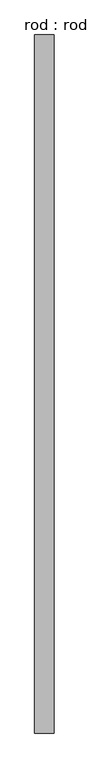
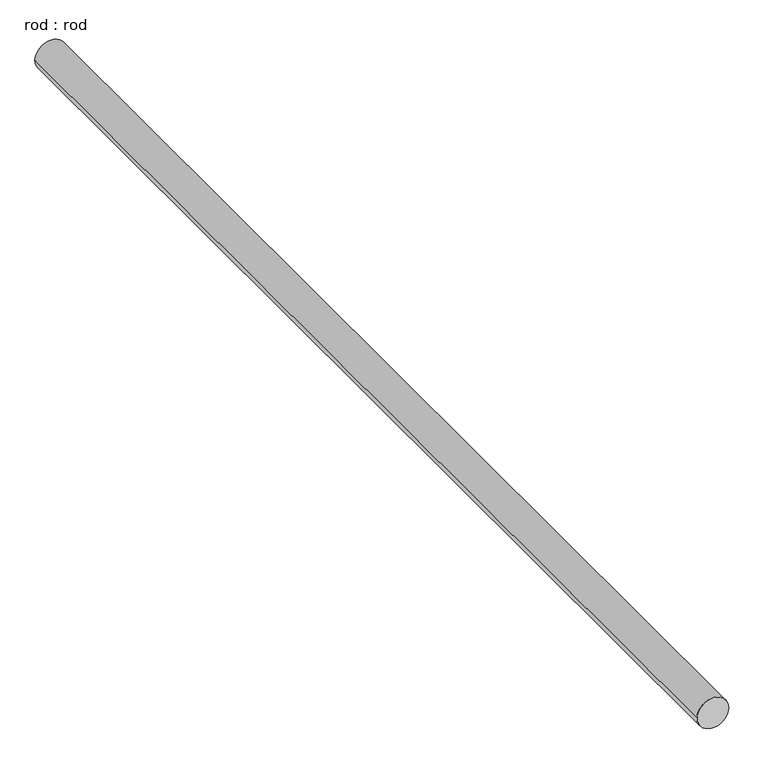
"""IFC4 building model written with IfcOpenShell, lengths in millimetres: proxy geometry, rod : rod."""

from ifc_helpers import new_model, si_unit, point, frame, frame_2d, origin, place, context, project, spatial, circle_curve, trimmed, segment, composite_curve, outline, extrude, source, transform, mapped, element, save


def rod_rod_e03d0b65(model_context):
    return source(origin(), model_context, "Body", "SweptSolid", [
        extrude(outline(composite_curve([segment(trimmed(circle_curve(frame_2d((0.0108462, 0.0)), 200.0), [point((0.0108462, 200.0))], [point((0.0108462, -200.0))], False, "CARTESIAN"), True, "CONTINUOUS"), segment(trimmed(circle_curve(frame_2d((0.0108462, 0.0)), 200.0), [point((0.0108462, -200.0))], [point((0.0108462, 200.0))], False, "CARTESIAN"), True, "CONTINUOUS")], self_intersect=False)), frame((0.0, -3159.948692, 0.0), z_axis=(0.0, 1.0, 0.0), x_axis=(0.0, 0.0, 1.0)), (0.0, 0.0, 1.0), 14505.3546148),
    ])


if __name__ == "__main__":
    model = new_model("IFC4")
    model_context = context("Model", 3, world=origin())
    ifc_project = project(units=[si_unit("LENGTHUNIT", "METRE", prefix="MILLI")], contexts=[model_context])
    site = spatial("IfcSite", under=ifc_project)
    building = spatial("IfcBuilding", under=site)
    placement = place(None, origin())
    rod_rod_shape = rod_rod_e03d0b65(model_context)
    element("IfcBuildingElementProxy", 1, Name="rod : rod", ObjectType="rod : rod", at=placement, inside=building, context=model_context, shape_type="MappedRepresentation", body=[
        mapped(rod_rod_shape, transform((0.0, 0.0, 0.0), x_axis=(1.0, 0.0, 0.0), y_axis=(0.0, 1.0, 0.0), z_axis=(0.0, 0.0, 1.0))),
    ])
    save(model, "model.ifc")

# Revit data of these elements
# Type "rod : rod"
#   Default Elevation = 0
